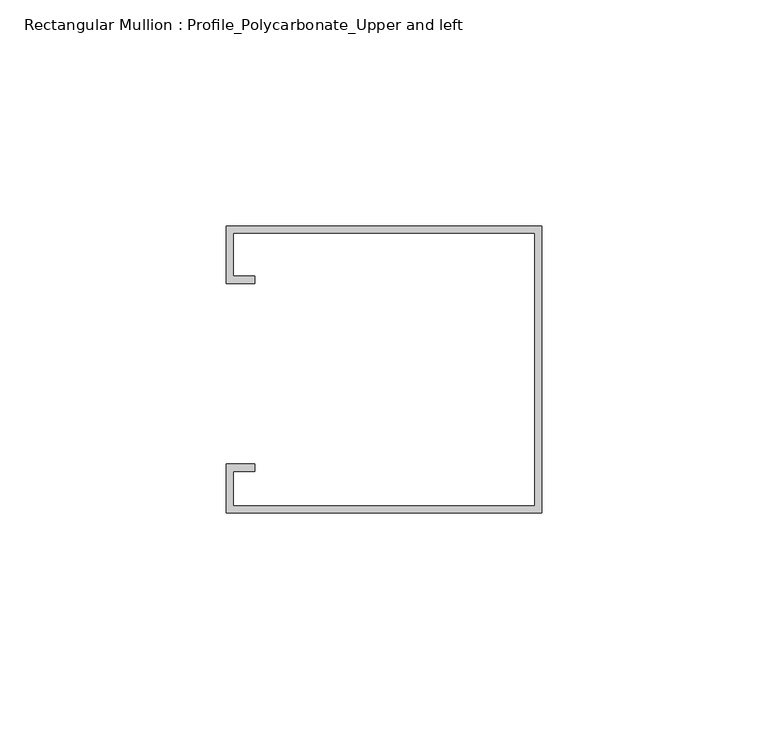
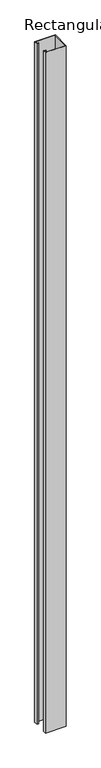
"""IFC4 building model written with IfcOpenShell, lengths in millimetres: member geometry, Rectangular Mullion : Profile_Polycarbonate_Upper and left."""

from ifc_helpers import new_model, si_unit, frame, origin, place, context, project, spatial, polyline, outline, extrude, source, transform, mapped, element, save


def rectangular_mullion_profile_polycarbonate_upper_and_left_1c393043(model_context):
    return source(origin(), model_context, "Body", "SweptSolid", [
        extrude(outline(polyline([(0.0, 32.7), (0.0, -30.8), (-69.85, -30.8), (-69.85, -20.0), (-63.5, -20.0), (-63.5, -21.5875), (-68.2625, -21.5875), (-68.2625, -29.2125), (-1.5875, -29.2125), (-1.5875, 31.1125), (-68.2625, 31.1125), (-68.2625, 21.5875), (-63.5, 21.5875), (-63.5, 20.0), (-69.85, 20.0), (-69.85, 32.7), (0.0, 32.7)])), frame((0.0, 0.0, -2438.4), z_axis=(0.0, 0.0, 1.0), x_axis=(1.0, 0.0, 0.0)), (0.0, 0.0, 1.0), 2438.4),
    ])


if __name__ == "__main__":
    model = new_model("IFC4")
    model_context = context("Model", 3, world=origin())
    ifc_project = project(units=[si_unit("LENGTHUNIT", "METRE", prefix="MILLI")], contexts=[model_context])
    site = spatial("IfcSite", under=ifc_project)
    building = spatial("IfcBuilding", under=site)
    placement = place(None, origin())
    rectangular_mullion_profile_polycarbonate_upper_and_left_shape = rectangular_mullion_profile_polycarbonate_upper_and_left_1c393043(model_context)
    element("IfcMember", 1, ObjectType="Rectangular Mullion : Profile_Polycarbonate_Upper and left", at=placement, inside=building, context=model_context, shape_type="MappedRepresentation", body=[
        mapped(rectangular_mullion_profile_polycarbonate_upper_and_left_shape, transform((0.0, 0.0, 0.0), x_axis=(1.0, 0.0, 0.0), y_axis=(0.0, 1.0, 0.0), z_axis=(0.0, 0.0, 1.0))),
    ])
    save(model, "model.ifc")

# Revit data of these elements
# Type "Rectangular Mullion : Profile_Polycarbonate_Upper and left"
#   built-in parameter 1007322 = 0.208333 (stored number, unit not read)
#   built-in parameter 1007321 = 0.00520833 (stored number, unit not read)
#   built-in parameter 1007320 = 0 (stored number, unit not read)
# Element 1 (IfcMember, "Rectangular Mullion : Profile_Polycarbonate_Upper and left")
#   Materials on its faces: "Aluminum"
# Materials
#   "Aluminum": class "Metal", colour RGB 244 244 244, transparency 0, Description = "Aluminum 6061", Cost = 0
